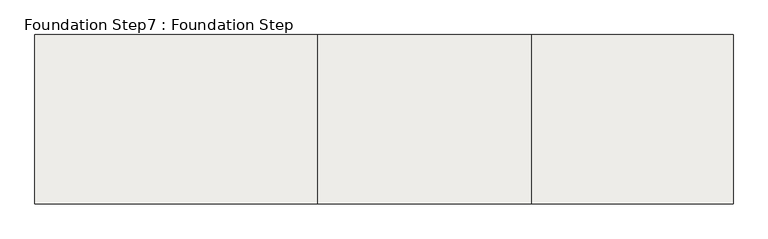
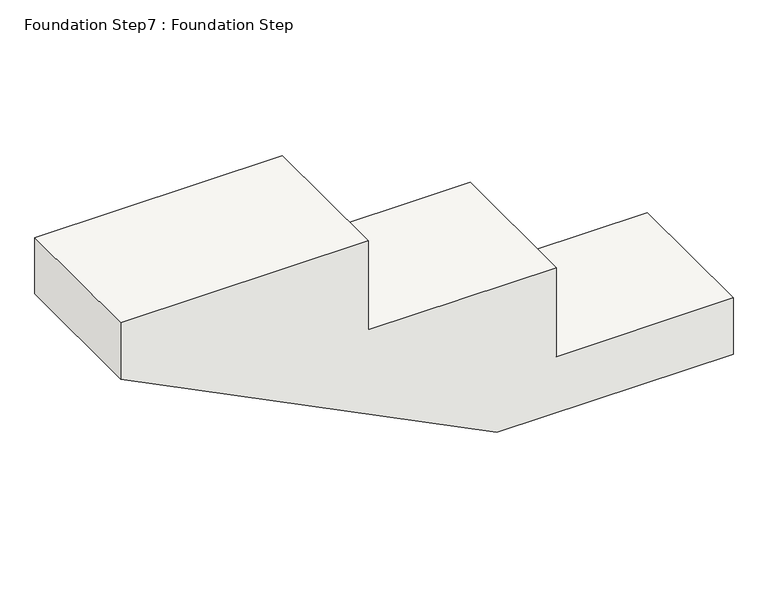
"""IFC4 building model written with IfcOpenShell, lengths in millimetres: slab geometry, Foundation Step7 : Foundation Step."""

from ifc_helpers import new_model, si_unit, frame, origin, place, context, project, spatial, polyline, outline, extrude, source, transform, mapped, element, save


def foundation_step7_foundation_step_1080ab70(model_context):
    return source(origin(), model_context, "Body", "SweptSolid", [
        extrude(outline(polyline([(-1092.2, -52957.4600821), (-1397.0, -52957.4600821), (-2362.2, -51027.0600821), (-2362.2, -49814.2100821), (-2057.4, -49814.2100821), (-2057.4, -50722.2600821), (-1574.8, -50722.2600821), (-1574.8, -51687.4600821), (-1092.2, -51687.4600821), (-1092.2, -52957.4600821)])), frame((0.0, -10673.0231529, 0.0), z_axis=(0.0, 1.0, 0.0), x_axis=(0.0, 0.0, 1.0)), (0.0, 0.0, 1.0), 762.0),
    ])


if __name__ == "__main__":
    model = new_model("IFC4")
    model_context = context("Model", 3, world=origin())
    ifc_project = project(units=[si_unit("LENGTHUNIT", "METRE", prefix="MILLI")], contexts=[model_context])
    site = spatial("IfcSite", under=ifc_project)
    building = spatial("IfcBuilding", under=site)
    placement = place(None, origin())
    foundation_step7_foundation_step_shape = foundation_step7_foundation_step_1080ab70(model_context)
    element("IfcSlab", 1, ObjectType="Foundation Step7 : Foundation Step", at=placement, inside=building, context=model_context, shape_type="MappedRepresentation", body=[
        mapped(foundation_step7_foundation_step_shape, transform((0.0, 0.0, 0.0), x_axis=(1.0, 0.0, 0.0), y_axis=(0.0, 1.0, 0.0), z_axis=(0.0, 0.0, 1.0))),
    ])
    save(model, "model.ifc")

# Revit data of these elements
# Type "Foundation Step7 : Foundation Step"
#   Structural Material = Concrete, Cast-in-Place gray
# Materials
#   "Concrete, Cast-in-Place gray": class "Concrete", colour RGB 192 192 192, transparency 0, Description = "Cast-in-place concrete", Cost = 0
